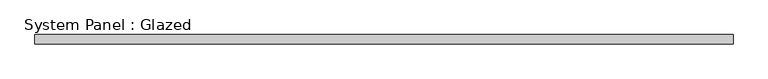
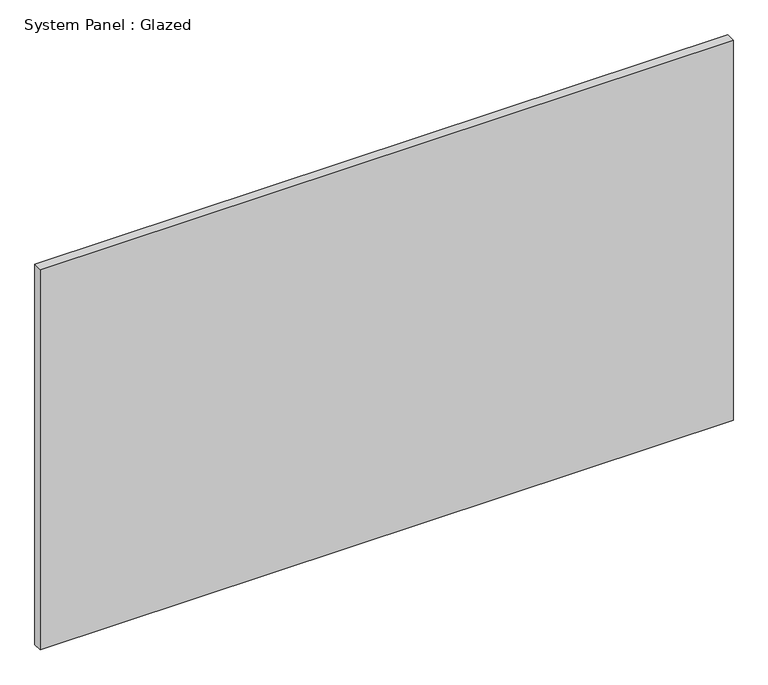
"""IFC4 building model written with IfcOpenShell, lengths in millimetres: plate geometry, System Panel : Glazed."""

from ifc_helpers import new_model, si_unit, origin, origin_with_axes, place, context, project, spatial, polyline, outline, extrude, source, transform, mapped, element, save


def system_panel_glazed_ac179f57(model_context):
    return source(origin(), model_context, "Body", "SweptSolid", [
        extrude(outline(polyline([(968.375, 19.05), (-968.375, 19.05), (-968.375, 44.45), (968.375, 44.45), (968.375, 19.05)])), origin_with_axes(), (0.0, 0.0, 1.0), 1123.95),
    ])


if __name__ == "__main__":
    model = new_model("IFC4")
    model_context = context("Model", 3, world=origin())
    ifc_project = project(units=[si_unit("LENGTHUNIT", "METRE", prefix="MILLI")], contexts=[model_context])
    site = spatial("IfcSite", under=ifc_project)
    building = spatial("IfcBuilding", under=site)
    placement = place(None, origin())
    system_panel_glazed_shape = system_panel_glazed_ac179f57(model_context)
    element("IfcPlate", 1, ObjectType="System Panel : Glazed", at=placement, inside=building, context=model_context, shape_type="MappedRepresentation", body=[
        mapped(system_panel_glazed_shape, transform((0.0, 0.0, 0.0), x_axis=(1.0, 0.0, 0.0), y_axis=(0.0, 1.0, 0.0), z_axis=(0.0, 0.0, 1.0))),
    ])
    save(model, "model.ifc")

# Revit data of these elements
# Element 1 (IfcPlate, "System Panel : Glazed")
#   Materials on its faces: "Glass"
# Materials
#   "Glass": class "Glass", colour RGB 0 128 192, transparency 0.75
